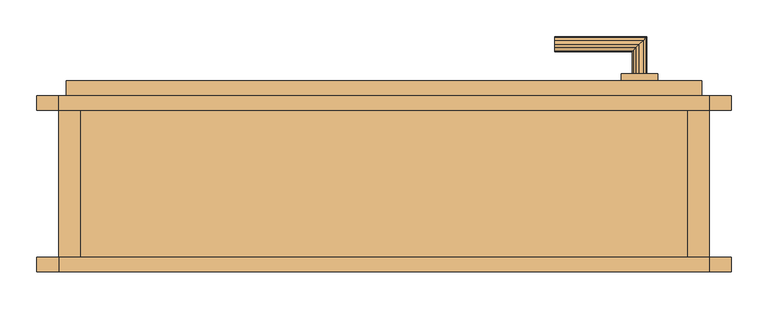
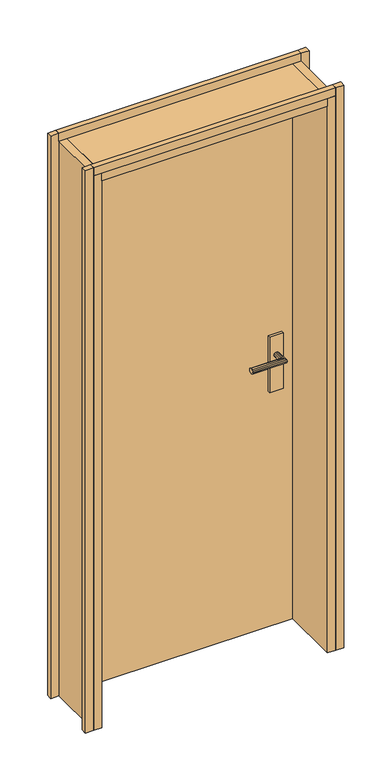
"""IFC4 building model written with IfcOpenShell, lengths in millimetres: door geometry, Tür."""

from ifc_helpers import new_model, si_unit, frame, origin, place, context, project, spatial, polyline, outline, extrude, faceted_brep, source, transform, mapped, element, save


def door_88c66588(model_context):
    return source(origin(), model_context, "Body", "SolidModel", [
        extrude(outline(polyline([(885.0, 220.0), (885.0, 200.0), (0.0, 200.0), (0.0, 220.0), (885.0, 220.0)])), frame((0.0, 0.0, 2285.0), z_axis=(0.0, 0.0, 1.0), x_axis=(1.0, 0.0, 0.0)), (0.0, 0.0, 1.0), 30.0),
        faceted_brep([(795.0, 250.0, 1198.660254), (790.0, 250.0, 1200.0), (785.0, 250.0, 1198.660254), (781.339746, 250.0, 1195.0), (780.0, 250.0, 1190.0), (781.339746, 250.0, 1185.0), (785.0, 250.0, 1181.339746), (790.0, 250.0, 1180.0), (795.0, 250.0, 1181.339746), (798.660254, 250.0, 1185.0), (800.0, 250.0, 1190.0), (798.660254, 250.0, 1195.0), (790.0, 290.0, 1200.0), (795.0, 295.0, 1198.660254), (798.660254, 298.660254, 1195.0), (800.0, 300.0, 1190.0), (798.660254, 298.660254, 1185.0), (795.0, 295.0, 1181.339746), (790.0, 290.0, 1180.0), (785.0, 285.0, 1181.339746), (781.339746, 281.339746, 1185.0), (780.0, 280.0, 1190.0), (781.339746, 281.339746, 1195.0), (785.0, 285.0, 1198.660254), (675.0, 285.0, 1198.660254), (675.0, 290.0, 1200.0), (675.0, 295.0, 1198.660254), (675.0, 298.660254, 1195.0), (675.0, 300.0, 1190.0), (675.0, 298.660254, 1185.0), (675.0, 295.0, 1181.339746), (675.0, 290.0, 1180.0), (675.0, 285.0, 1181.339746), (675.0, 281.339746, 1185.0), (675.0, 280.0, 1190.0), (675.0, 281.339746, 1195.0)], [[[0, 1, 2, 3, 4, 5, 6, 7, 8, 9, 10, 11]], [[12, 1, 0, 13]], [[13, 0, 11, 14]], [[14, 11, 10, 15]], [[15, 10, 9, 16]], [[16, 9, 8, 17]], [[17, 8, 7, 18]], [[18, 7, 6, 19]], [[19, 6, 5, 20]], [[20, 5, 4, 21]], [[21, 4, 3, 22]], [[22, 3, 2, 23]], [[23, 2, 1, 12]], [[24, 25, 26, 27, 28, 29, 30, 31, 32, 33, 34, 35]], [[25, 12, 13, 26]], [[26, 13, 14, 27]], [[27, 14, 15, 28]], [[28, 15, 16, 29]], [[29, 16, 17, 30]], [[30, 17, 18, 31]], [[31, 18, 19, 32]], [[32, 19, 20, 33]], [[33, 20, 21, 34]], [[34, 21, 22, 35]], [[35, 22, 23, 24]], [[24, 23, 12, 25]]]),
        extrude(outline(polyline([(0.0, -20.0), (-30.0, -20.0), (-30.0, 0.0), (0.0, 0.0), (0.0, -20.0)])), frame((0.0, 0.0, 140.0), z_axis=(0.0, 0.0, 1.0), x_axis=(1.0, 0.0, 0.0)), (0.0, 0.0, 1.0), 2175.0),
        extrude(outline(polyline([(765.0, 200.0), (815.0, 200.0), (815.0, 190.0), (765.0, 190.0), (765.0, 200.0)])), frame((0.0, 0.0, 1050.0), z_axis=(0.0, 0.0, 1.0), x_axis=(1.0, 0.0, 0.0)), (0.0, 0.0, 1.0), 215.0),
        extrude(outline(polyline([(885.0, 0.0), (885.0, -20.0), (0.0, -20.0), (0.0, 0.0), (885.0, 0.0)])), frame((0.0, 0.0, 2285.0), z_axis=(0.0, 0.0, 1.0), x_axis=(1.0, 0.0, 0.0)), (0.0, 0.0, 1.0), 30.0),
        extrude(outline(polyline([(875.0, 240.0), (875.0, 200.0), (10.0, 200.0), (10.0, 240.0), (875.0, 240.0)])), frame((0.0, 0.0, 140.0), z_axis=(0.0, 0.0, 1.0), x_axis=(1.0, 0.0, 0.0)), (0.0, 0.0, 1.0), 2135.0),
        extrude(outline(polyline([(915.0, 0.0), (915.0, -20.0), (885.0, -20.0), (885.0, 0.0), (915.0, 0.0)])), frame((0.0, 0.0, 140.0), z_axis=(0.0, 0.0, 1.0), x_axis=(1.0, 0.0, 0.0)), (0.0, 0.0, 1.0), 2175.0),
        extrude(outline(polyline([(0.0, 200.0), (-30.0, 200.0), (-30.0, 220.0), (0.0, 220.0), (0.0, 200.0)])), frame((0.0, 0.0, 140.0), z_axis=(0.0, 0.0, 1.0), x_axis=(1.0, 0.0, 0.0)), (0.0, 0.0, 1.0), 2175.0),
        extrude(outline(polyline([(855.0, 220.0), (855.0, -20.0), (30.0, -20.0), (30.0, 220.0), (855.0, 220.0)])), frame((0.0, 0.0, 2255.0), z_axis=(0.0, 0.0, 1.0), x_axis=(1.0, 0.0, 0.0)), (0.0, 0.0, 1.0), 30.0),
        extrude(outline(polyline([(815.0, 250.0), (815.0, 240.0), (765.0, 240.0), (765.0, 250.0), (815.0, 250.0)])), frame((0.0, 0.0, 1050.0), z_axis=(0.0, 0.0, 1.0), x_axis=(1.0, 0.0, 0.0)), (0.0, 0.0, 1.0), 215.0),
        extrude(outline(polyline([(885.0, 220.0), (885.0, -20.0), (855.0, -20.0), (855.0, 220.0), (885.0, 220.0)])), frame((0.0, 0.0, 140.0), z_axis=(0.0, 0.0, 1.0), x_axis=(1.0, 0.0, 0.0)), (0.0, 0.0, 1.0), 2145.0),
        extrude(outline(polyline([(30.0, 220.0), (30.0, -20.0), (0.0, -20.0), (0.0, 220.0), (30.0, 220.0)])), frame((0.0, 0.0, 140.0), z_axis=(0.0, 0.0, 1.0), x_axis=(1.0, 0.0, 0.0)), (0.0, 0.0, 1.0), 2145.0),
        extrude(outline(polyline([(915.0, 220.0), (915.0, 200.0), (885.0, 200.0), (885.0, 220.0), (915.0, 220.0)])), frame((0.0, 0.0, 140.0), z_axis=(0.0, 0.0, 1.0), x_axis=(1.0, 0.0, 0.0)), (0.0, 0.0, 1.0), 2175.0),
        faceted_brep([(785.0, 190.0, 1198.660254), (790.0, 190.0, 1200.0), (795.0, 190.0, 1198.660254), (798.660254, 190.0, 1195.0), (800.0, 190.0, 1190.0), (798.660254, 190.0, 1185.0), (795.0, 190.0, 1181.339746), (790.0, 190.0, 1180.0), (785.0, 190.0, 1181.339746), (781.339746, 190.0, 1185.0), (780.0, 190.0, 1190.0), (781.339746, 190.0, 1195.0), (790.0, 150.0, 1200.0), (795.0, 145.0, 1198.660254), (798.660254, 141.339746, 1195.0), (800.0, 140.0, 1190.0), (798.660254, 141.339746, 1185.0), (795.0, 145.0, 1181.339746), (790.0, 150.0, 1180.0), (785.0, 155.0, 1181.339746), (781.339746, 158.660254, 1185.0), (780.0, 160.0, 1190.0), (781.339746, 158.660254, 1195.0), (785.0, 155.0, 1198.660254), (675.0, 145.0, 1198.660254), (675.0, 150.0, 1200.0), (675.0, 155.0, 1198.660254), (675.0, 158.660254, 1195.0), (675.0, 160.0, 1190.0), (675.0, 158.660254, 1185.0), (675.0, 155.0, 1181.339746), (675.0, 150.0, 1180.0), (675.0, 145.0, 1181.339746), (675.0, 141.339746, 1185.0), (675.0, 140.0, 1190.0), (675.0, 141.339746, 1195.0)], [[[0, 1, 2, 3, 4, 5, 6, 7, 8, 9, 10, 11]], [[2, 1, 12, 13]], [[3, 2, 13, 14]], [[4, 3, 14, 15]], [[5, 4, 15, 16]], [[6, 5, 16, 17]], [[7, 6, 17, 18]], [[8, 7, 18, 19]], [[9, 8, 19, 20]], [[10, 9, 20, 21]], [[11, 10, 21, 22]], [[0, 11, 22, 23]], [[1, 0, 23, 12]], [[24, 25, 26, 27, 28, 29, 30, 31, 32, 33, 34, 35]], [[13, 12, 25, 24]], [[14, 13, 24, 35]], [[15, 14, 35, 34]], [[16, 15, 34, 33]], [[17, 16, 33, 32]], [[18, 17, 32, 31]], [[19, 18, 31, 30]], [[20, 19, 30, 29]], [[21, 20, 29, 28]], [[22, 21, 28, 27]], [[23, 22, 27, 26]], [[12, 23, 26, 25]]]),
    ])


if __name__ == "__main__":
    model = new_model("IFC4")
    model_context = context("Model", 3, world=origin())
    ifc_project = project(units=[si_unit("LENGTHUNIT", "METRE", prefix="MILLI")], contexts=[model_context])
    site = spatial("IfcSite", under=ifc_project)
    building = spatial("IfcBuilding", under=site)
    placement = place(None, origin())
    door_shape = door_88c66588(model_context)
    element("IfcDoor", 1, ObjectType="Tür", at=placement, inside=building, context=model_context, shape_type="MappedRepresentation", body=[
        mapped(door_shape, transform((0.0, 0.0, 0.0), x_axis=(1.0, 0.0, 0.0), y_axis=(0.0, 1.0, 0.0), z_axis=(0.0, 0.0, 1.0))),
    ])
    save(model, "model.ifc")

# Revit data of these elements
# Type "Tür"
#   Type Mark = "44"
# Element 1 (IfcDoor, "Tür")
#   Materials on its faces: "tuer_beschlag", "tuer_holzzarge"
# Materials
#   "tuer_beschlag": class "Unassigned", colour RGB 128 128 128, transparency 0
#   "tuer_holzzarge": class "Unassigned", colour RGB 255 255 255, transparency 0
